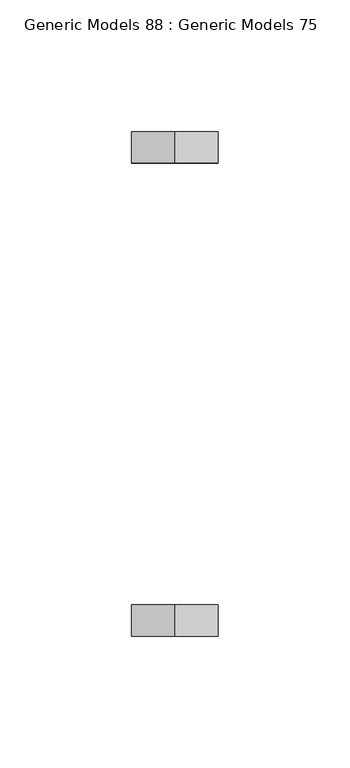
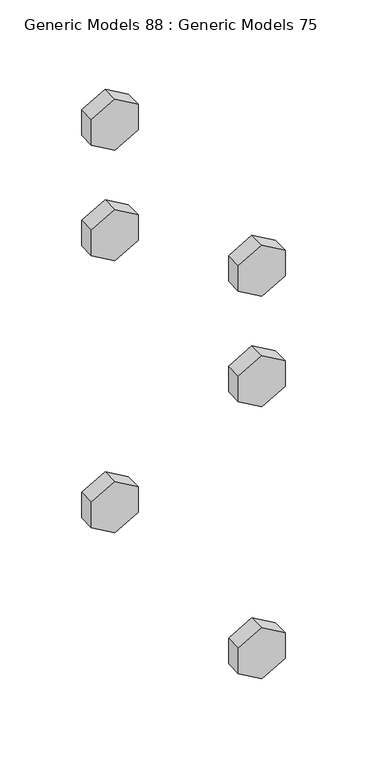
"""IFC4 building model written with IfcOpenShell, lengths in millimetres: proxy geometry, Generic Models 88 : Generic Models 75."""

from ifc_helpers import new_model, si_unit, frame, origin, place, context, project, spatial, polyline, outline, extrude, source, transform, mapped, element, save


def generic_models_88_generic_models_75_4cb196d4(model_context):
    return source(origin(), model_context, "Body", "SweptSolid", [
        extrude(outline(polyline([(271427.575, 31991.9073871), (271446.625, 31991.9073871), (271456.15, 31975.4096032), (271446.625, 31958.9118192), (271427.575, 31958.9118192), (271418.05, 31975.4096032), (271427.575, 31991.9073871)])), frame((0.0, 35193.7770442, 0.0), z_axis=(0.0, 1.0, 0.0), x_axis=(0.0, 0.0, 1.0)), (0.0, 0.0, 1.0), 11.90625),
        extrude(outline(polyline([(271713.325, 31991.9073871), (271732.375, 31991.9073871), (271741.9, 31975.4096032), (271732.375, 31958.9118192), (271713.325, 31958.9118192), (271703.8, 31975.4096032), (271713.325, 31991.9073871)])), frame((0.0, 35193.7770442, 0.0), z_axis=(0.0, 1.0, 0.0), x_axis=(0.0, 0.0, 1.0)), (0.0, 0.0, 1.0), 11.90625),
        extrude(outline(polyline([(271630.775, 31991.9073871), (271649.825, 31991.9073871), (271659.35, 31975.4096032), (271649.825, 31958.9118192), (271630.775, 31958.9118192), (271621.25, 31975.4096032), (271630.775, 31991.9073871)])), frame((0.0, 35193.7770442, 0.0), z_axis=(0.0, 1.0, 0.0), x_axis=(0.0, 0.0, 1.0)), (0.0, 0.0, 1.0), 11.90625),
        extrude(outline(polyline([(271630.775, 31991.9073871), (271649.825, 31991.9073871), (271659.35, 31975.4096032), (271649.825, 31958.9118192), (271630.775, 31958.9118192), (271621.25, 31975.4096032), (271630.775, 31991.9073871)])), frame((0.0, 35373.5614192, 0.0), z_axis=(0.0, 1.0, 0.0), x_axis=(0.0, 0.0, 1.0)), (0.0, 0.0, 1.0), 11.90625),
        extrude(outline(polyline([(271427.575, 31991.9073871), (271446.625, 31991.9073871), (271456.15, 31975.4096032), (271446.625, 31958.9118192), (271427.575, 31958.9118192), (271418.05, 31975.4096032), (271427.575, 31991.9073871)])), frame((0.0, 35373.5614192, 0.0), z_axis=(0.0, 1.0, 0.0), x_axis=(0.0, 0.0, 1.0)), (0.0, 0.0, 1.0), 11.90625),
        extrude(outline(polyline([(271713.325, 31991.9073871), (271732.375, 31991.9073871), (271741.9, 31975.4096032), (271732.375, 31958.9118192), (271713.325, 31958.9118192), (271703.8, 31975.4096032), (271713.325, 31991.9073871)])), frame((0.0, 35373.5614192, 0.0), z_axis=(0.0, 1.0, 0.0), x_axis=(0.0, 0.0, 1.0)), (0.0, 0.0, 1.0), 11.90625),
    ])


if __name__ == "__main__":
    model = new_model("IFC4")
    model_context = context("Model", 3, world=origin())
    ifc_project = project(units=[si_unit("LENGTHUNIT", "METRE", prefix="MILLI")], contexts=[model_context])
    site = spatial("IfcSite", under=ifc_project)
    building = spatial("IfcBuilding", under=site)
    placement = place(None, origin())
    generic_models_88_generic_models_75_shape = generic_models_88_generic_models_75_4cb196d4(model_context)
    element("IfcBuildingElementProxy", 1, Name="Generic Models 88 : Generic Models 75", ObjectType="Generic Models 88 : Generic Models 75", at=placement, inside=building, context=model_context, shape_type="MappedRepresentation", body=[
        mapped(generic_models_88_generic_models_75_shape, transform((0.0, 0.0, 0.0), x_axis=(1.0, 0.0, 0.0), y_axis=(0.0, 1.0, 0.0), z_axis=(0.0, 0.0, 1.0))),
    ])
    save(model, "model.ifc")
